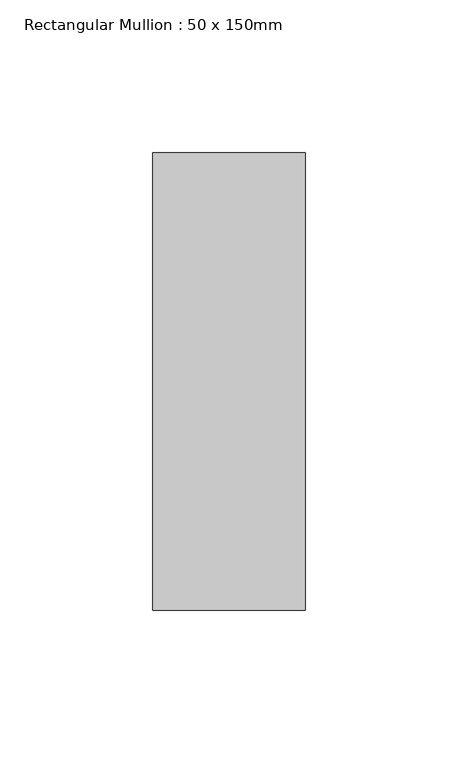
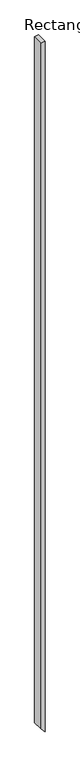
"""IFC4 building model written with IfcOpenShell, lengths in millimetres: member geometry, Rectangular Mullion : 50 x 150mm."""

from ifc_helpers import new_model, si_unit, frame, origin, place, context, project, spatial, polyline, outline, extrude, source, transform, mapped, element, save


def rectangular_mullion_50_x_150mm_3d64617b(model_context):
    return source(origin(), model_context, "Body", "SweptSolid", [
        extrude(outline(polyline([(0.0, 0.0), (-11.7094446, -50.0), (-9724.6362561, -50.0), (-9783.1614006, 0.0), (0.0, 0.0)])), frame((0.0, -75.0, 0.0), z_axis=(0.0, 1.0, 0.0), x_axis=(0.0, 0.0, 1.0)), (0.0, 0.0, 1.0), 150.0),
    ])


if __name__ == "__main__":
    model = new_model("IFC4")
    model_context = context("Model", 3, world=origin())
    ifc_project = project(units=[si_unit("LENGTHUNIT", "METRE", prefix="MILLI")], contexts=[model_context])
    site = spatial("IfcSite", under=ifc_project)
    building = spatial("IfcBuilding", under=site)
    placement = place(None, origin())
    rectangular_mullion_50_x_150mm_shape = rectangular_mullion_50_x_150mm_3d64617b(model_context)
    element("IfcMember", 1, ObjectType="Rectangular Mullion : 50 x 150mm", at=placement, inside=building, context=model_context, shape_type="MappedRepresentation", body=[
        mapped(rectangular_mullion_50_x_150mm_shape, transform((0.0, 0.0, 0.0), x_axis=(1.0, 0.0, 0.0), y_axis=(0.0, 1.0, 0.0), z_axis=(0.0, 0.0, 1.0))),
    ])
    save(model, "model.ifc")

# Revit data of these elements
# Type "Rectangular Mullion : 50 x 150mm"
#   built-in parameter 1007304 = 0.492126 (stored number, unit not read)
#   built-in parameter 1007301 = 0.082021 (stored number, unit not read)
#   built-in parameter 1007300 = 0.082021 (stored number, unit not read)
# Element 1 (IfcMember, "Rectangular Mullion : 50 x 150mm")
#   Materials on its faces: "Metal - Aluminium"
# Materials
#   "Metal - Aluminium": class "Metal", colour RGB 247 247 247, transparency 0
